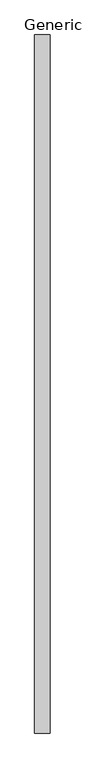
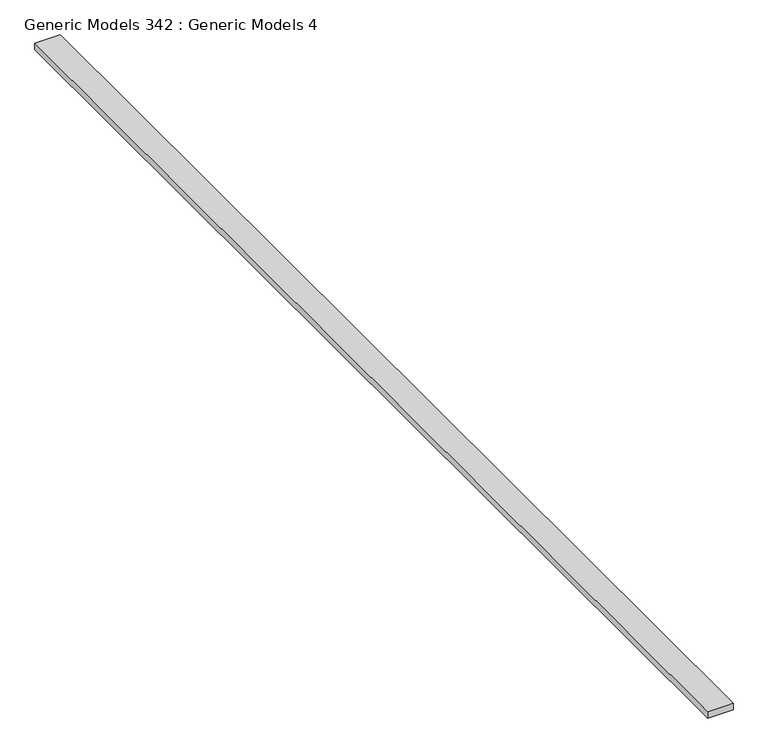
"""IFC4 building model written with IfcOpenShell, lengths in millimetres: proxy geometry, Generic Models 342 : Generic Models 4."""

import ifcopenshell
import ifcopenshell.guid

model = None  # the IFC model being written
_history = None  # IfcOwnerHistory: only IFC2X3 demands one
_inside = {}  # id of a spatial element -> (the spatial element, [elements in it])
_under = {}  # id of a project, library or spatial element -> (it, [spatial elements below it])
_declared = {}  # id of a project -> (the project, [libraries it declares])
_typed = {}  # id of a type object -> (the type object, [elements of that type])
_made_of = {}  # id of a material, layer set ... -> (it, [elements and type objects made of it])


def new_model(schema):
    """Start an empty IFC model of exactly this schema.

    Asked for "IFC4X3", IfcOpenShell would pick the latest addendum, in which some entities
    have other attributes; the version numbers below select the first issue.
    IFC2X3 requires an IfcOwnerHistory on every rooted entity: one is made here for all.
    """
    global model, _history
    if schema == "IFC4X3":
        model = ifcopenshell.file(schema_version=(4, 3, 0, 0))
    else:
        model = ifcopenshell.file(schema=schema)
    _inside.clear()
    _under.clear()
    _declared.clear()
    _typed.clear()
    _made_of.clear()
    _history = None
    if model.schema == "IFC2X3":
        org = make("IfcOrganization", Name="unknown")
        user = make(
            "IfcPersonAndOrganization",
            ThePerson=make("IfcPerson", FamilyName="unknown"),
            TheOrganization=org,
        )
        app = make(
            "IfcApplication",
            ApplicationDeveloper=org,
            Version="unknown",
            ApplicationFullName="unknown",
            ApplicationIdentifier="unknown",
        )
        _history = make(
            "IfcOwnerHistory",
            OwningUser=user,
            OwningApplication=app,
            ChangeAction="ADDED",
            CreationDate=0,
        )
    return model


def make(cls, **values):
    """One entity of the class cls with the attributes given. An attribute that is None is left unset."""
    return model.create_entity(
        cls, **{name: value for name, value in values.items() if value is not None}
    )


def rooted(cls, **values):
    """An entity with a GlobalId (a new one), such as an element, a storey or a relation."""
    return make(cls, GlobalId=ifcopenshell.guid.new(), OwnerHistory=_history, **values)


def si_unit(unit_type, name, prefix=None):
    """IfcSIUnit, for example si_unit("LENGTHUNIT", "METRE", prefix="MILLI")."""
    return make("IfcSIUnit", UnitType=unit_type, Prefix=prefix, Name=name)


def assignment(units):
    """IfcUnitAssignment: the units of a project."""
    return None if units is None else make("IfcUnitAssignment", Units=units)


def point(xyz):
    """IfcCartesianPoint."""
    return None if xyz is None else make("IfcCartesianPoint", Coordinates=xyz)


def direction(xyz):
    """IfcDirection."""
    return None if xyz is None else make("IfcDirection", DirectionRatios=xyz)


def frame(location, z_axis=None, x_axis=None):
    """IfcAxis2Placement3D, a coordinate frame: its origin and axes. An axis left out is left unset."""
    return make(
        "IfcAxis2Placement3D",
        Location=point(location),
        Axis=direction(z_axis),
        RefDirection=direction(x_axis),
    )


def origin():
    """The frame at (0, 0, 0) with its axes left unset."""
    return frame((0.0, 0.0, 0.0))


def place(relative_to, where):
    """IfcLocalPlacement: puts the frame where relative to a parent placement (None: the world)."""
    return make(
        "IfcLocalPlacement", PlacementRelTo=relative_to, RelativePlacement=where
    )


def context(
    kind, dimensions, precision=None, world=None, true_north=None, identifier=None
):
    """IfcGeometricRepresentationContext, for example the 3D "Model" context."""
    return make(
        "IfcGeometricRepresentationContext",
        ContextIdentifier=identifier,
        ContextType=kind,
        CoordinateSpaceDimension=dimensions,
        Precision=precision,
        WorldCoordinateSystem=world,
        TrueNorth=true_north,
    )


def project(units=None, contexts=None):
    """IfcProject with its units and contexts."""
    return rooted(
        "IfcProject",
        Name="project",
        RepresentationContexts=contexts,
        UnitsInContext=assignment(units),
    )


def spatial(cls, under=None, at=None, **own):
    """A site, building, storey or space (cls), placed at a placement, below another one or the project."""
    s = rooted(cls, ObjectPlacement=at, **own)
    if under is not None:
        _under.setdefault(under.id(), (under, []))[1].append(s)
    return s


def polyline(points):
    """IfcPolyline through the points."""
    return make("IfcPolyline", Points=[point(p) for p in points])


def outline(outer, holes=None, kind="AREA"):
    """IfcArbitraryClosedProfileDef: a profile drawn as a closed curve; with holes, ...WithVoids."""
    if holes is None:
        return make("IfcArbitraryClosedProfileDef", ProfileType=kind, OuterCurve=outer)
    return make(
        "IfcArbitraryProfileDefWithVoids",
        ProfileType=kind,
        OuterCurve=outer,
        InnerCurves=holes,
    )


def extrude(swept, where, along, depth):
    """IfcExtrudedAreaSolid: the profile swept, set in the frame where, extruded along a direction by depth."""
    return make(
        "IfcExtrudedAreaSolid",
        SweptArea=swept,
        Position=where,
        ExtrudedDirection=direction(along),
        Depth=depth,
    )


def shape(context_of_items, identifier, shape_type, items):
    """IfcShapeRepresentation: the items that make up one representation, for example the "Body"."""
    return make(
        "IfcShapeRepresentation",
        ContextOfItems=context_of_items,
        RepresentationIdentifier=identifier,
        RepresentationType=shape_type,
        Items=items,
    )


def source(mapping_origin, context_of_items, identifier, shape_type, items):
    """IfcRepresentationMap: a shape defined once, which mapped items show again and again."""
    return make(
        "IfcRepresentationMap",
        MappingOrigin=mapping_origin,
        MappedRepresentation=shape(context_of_items, identifier, shape_type, items),
    )


def transform(
    local_origin,
    x_axis=None,
    y_axis=None,
    z_axis=None,
    scale=None,
    scale2=None,
    scale3=None,
    uniform=True,
):
    """IfcCartesianTransformationOperator3D, or its non-uniform kind. x_axis, y_axis, z_axis: its Axis1, 2, 3."""
    if uniform:
        return make(
            "IfcCartesianTransformationOperator3D",
            Axis1=direction(x_axis),
            Axis2=direction(y_axis),
            LocalOrigin=point(local_origin),
            Scale=scale,
            Axis3=direction(z_axis),
        )
    return make(
        "IfcCartesianTransformationOperator3DnonUniform",
        Axis1=direction(x_axis),
        Axis2=direction(y_axis),
        LocalOrigin=point(local_origin),
        Scale=scale,
        Axis3=direction(z_axis),
        Scale2=scale2,
        Scale3=scale3,
    )


def mapped(mapping_source, mapping_target):
    """IfcMappedItem: shows the shape of a source again, moved by a transform."""
    return make(
        "IfcMappedItem", MappingSource=mapping_source, MappingTarget=mapping_target
    )


def made_of(thing, what):
    """Note that an element or type object is made of a material, layer set ...; save() writes the relation."""
    if what is not None:
        _made_of.setdefault(what.id(), (what, []))[1].append(thing)
    return thing


def element(
    cls,
    number,
    at=None,
    inside=None,
    cuts=None,
    type_object=None,
    material=None,
    context=None,
    identifier="Body",
    shape_type=None,
    held_by="IfcProductDefinitionShape",
    body=None,
    shapes=None,
    **own,
):
    """One element of the class cls, such as IfcWall. Its Tag is "e" and its number.

    at: its placement. inside: the storey or other place that contains it. cuts: it is an
    opening in that element (IfcRelVoidsElement). A single representation is given by context,
    identifier, shape_type and body (its items); several are given by shapes. held_by: the class
    of the entity that holds the representations. save() writes the other relations.
    """
    e = rooted(cls, Tag="e%d" % number, ObjectPlacement=at, **own)
    if body is not None:
        shapes = [shape(context, identifier, shape_type, body)]
    if shapes is not None:
        e.Representation = make(held_by, Representations=shapes)
    if inside is not None:
        _inside.setdefault(inside.id(), (inside, []))[1].append(e)
    if cuts is not None:
        rooted(
            "IfcRelVoidsElement", RelatingBuildingElement=cuts, RelatedOpeningElement=e
        )
    if type_object is not None:
        _typed.setdefault(type_object.id(), (type_object, []))[1].append(e)
    return made_of(e, material)


def aggregate(whole, parts):
    """IfcRelAggregates: a whole, such as a stair, and the parts it consists of."""
    return rooted("IfcRelAggregates", RelatingObject=whole, RelatedObjects=parts)


def save(model, path):
    """Write the relations noted so far, then the file.

    IfcRelAggregates (storeys below a building ...), IfcRelContainedInSpatialStructure (elements
    in a storey), IfcRelDefinesByType, IfcRelAssociatesMaterial and IfcRelDeclares: one each for
    every whole, place, type object, material and project.
    """
    for whole, parts in _under.values():
        aggregate(whole, parts)
    for where, things in _inside.values():
        rooted(
            "IfcRelContainedInSpatialStructure",
            RelatedElements=things,
            RelatingStructure=where,
        )
    for kind, things in _typed.values():
        rooted("IfcRelDefinesByType", RelatedObjects=things, RelatingType=kind)
    for what, things in _made_of.values():
        rooted("IfcRelAssociatesMaterial", RelatedObjects=things, RelatingMaterial=what)
    for by, libraries in _declared.values():
        rooted("IfcRelDeclares", RelatingContext=by, RelatedDefinitions=libraries)
    model.write(path)


def generic_models_342_generic_models_4_2daae526(model_context):
    return source(origin(), model_context, "Body", "SweptSolid", [
        extrude(outline(polyline([(-6470.8236296, -6864.9230338), (-6610.5236296, -6864.9230338), (-6610.5236296, -464.1230338), (-6470.8236296, -464.1230338), (-6470.8236296, -6864.9230338)])), frame((0.0, 0.0, 126211.4078034), z_axis=(0.0, 0.0, 1.0), x_axis=(1.0, 0.0, 0.0)), (0.0, 0.0, 1.0), 37.1331966),
    ])


if __name__ == "__main__":
    model = new_model("IFC4")
    model_context = context("Model", 3, world=origin())
    ifc_project = project(units=[si_unit("LENGTHUNIT", "METRE", prefix="MILLI")], contexts=[model_context])
    site = spatial("IfcSite", under=ifc_project)
    building = spatial("IfcBuilding", under=site)
    placement = place(None, origin())
    generic_models_342_generic_models_4_shape = generic_models_342_generic_models_4_2daae526(model_context)
    element("IfcBuildingElementProxy", 1, Name="Generic Models 342 : Generic Models 4", ObjectType="Generic Models 342 : Generic Models 4", at=placement, inside=building, context=model_context, shape_type="MappedRepresentation", body=[
        mapped(generic_models_342_generic_models_4_shape, transform((0.0, 0.0, 0.0), x_axis=(1.0, 0.0, 0.0), y_axis=(0.0, 1.0, 0.0), z_axis=(0.0, 0.0, 1.0))),
    ])
    save(model, "model.ifc")

# Revit data of these elements
# Element 1 (IfcBuildingElementProxy, "Generic Models 342 : Generic Models 4")
#   Materials on its faces: "_2X BLOCKING AS REQUIRED"
# Materials
#   "_2X BLOCKING AS REQUIRED": class "Generic", colour RGB 177 130 114, transparency 0, Cost = 0
